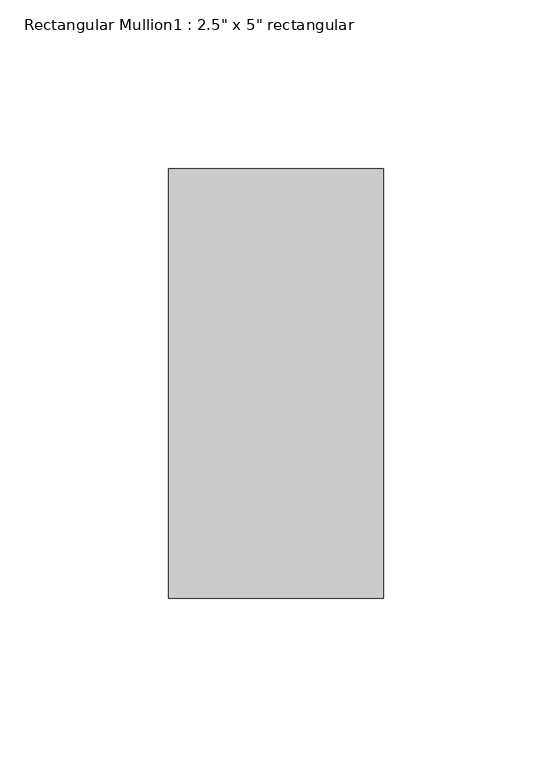
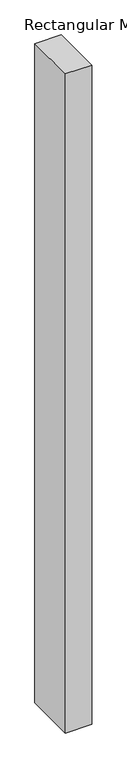
"""IFC4 building model written with IfcOpenShell, lengths in millimetres: member geometry."""

from ifc_helpers import new_model, si_unit, frame, origin, place, context, project, spatial, polyline, outline, extrude, source, transform, mapped, element, save


def member_062c1ce8(model_context):
    return source(origin(), model_context, "Body", "SweptSolid", [
        extrude(outline(polyline([(0.0, 63.5), (0.0, -63.5), (-63.5, -63.5), (-63.5, 63.5), (0.0, 63.5)])), frame((0.0, 0.0, -1676.4), z_axis=(0.0, 0.0, 1.0), x_axis=(1.0, 0.0, 0.0)), (0.0, 0.0, 1.0), 1676.4),
    ])


if __name__ == "__main__":
    model = new_model("IFC4")
    model_context = context("Model", 3, world=origin())
    ifc_project = project(units=[si_unit("LENGTHUNIT", "METRE", prefix="MILLI")], contexts=[model_context])
    site = spatial("IfcSite", under=ifc_project)
    building = spatial("IfcBuilding", under=site)
    placement = place(None, origin())
    member_shape = member_062c1ce8(model_context)
    element("IfcMember", 1, ObjectType="Rectangular Mullion1 : 2.5\" x 5\" rectangular", at=placement, inside=building, context=model_context, shape_type="MappedRepresentation", body=[
        mapped(member_shape, transform((0.0, 0.0, 0.0), x_axis=(1.0, 0.0, 0.0), y_axis=(0.0, 1.0, 0.0), z_axis=(0.0, 0.0, 1.0))),
    ])
    save(model, "model.ifc")

# Revit data of these elements
# Type "Rectangular Mullion1 : 2.5\" x 5\" rectangular"
#   built-in parameter 1007304 = 0.416667 (stored number, unit not read)
#   built-in parameter 1007301 = 0.104167 (stored number, unit not read)
#   built-in parameter 1007300 = 0.104167 (stored number, unit not read)
# Element 1 (IfcMember, "Rectangular Mullion1 : 2.5\" x 5\" rectangular")
#   Materials on its faces: "support-frame"
# Materials
#   "support-frame": class "Unassigned", colour RGB 233 233 233, transparency 0, Cost = 0
